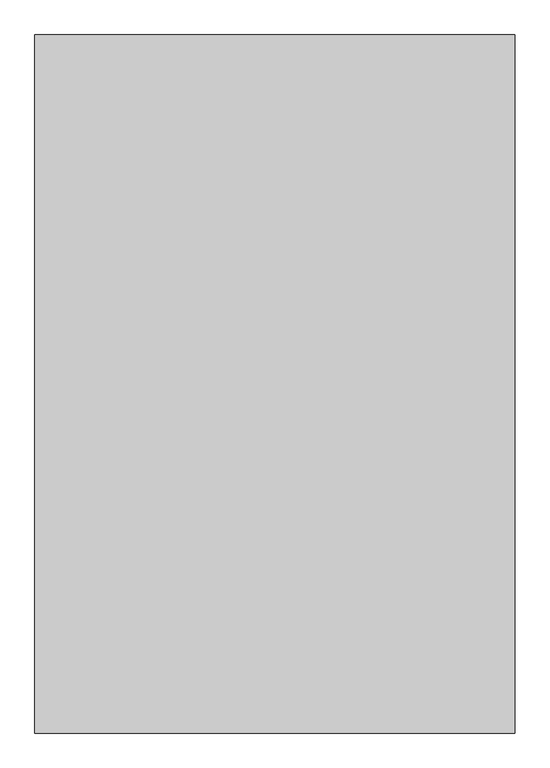
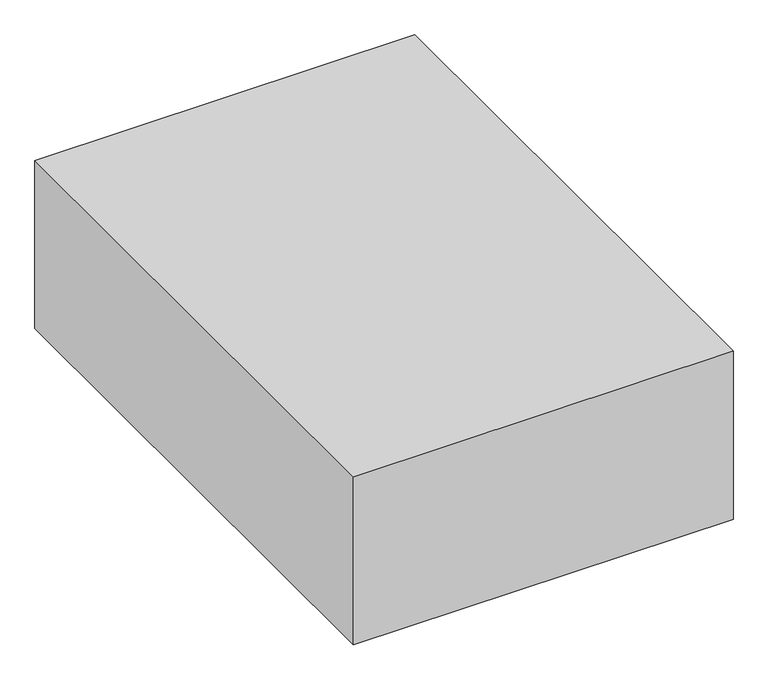
"""IFC4 building model written with IfcOpenShell, lengths in millimetres: proxy geometry, Space Planning Box_hec : Space Planning Box_hec."""

from ifc_helpers import new_model, si_unit, origin, origin_with_axes, place, context, project, spatial, polyline, outline, extrude, source, transform, mapped, element, save


def generic_models_21711933(model_context):
    return source(origin(), model_context, "Body", "SweptSolid", [
        extrude(outline(polyline([(6400.0, 9300.0), (6400.0, -9300.0), (-6400.0, -9300.0), (-6400.0, 9300.0), (6400.0, 9300.0)])), origin_with_axes(), (0.0, 0.0, 1.0), 6000.0),
    ])


if __name__ == "__main__":
    model = new_model("IFC4")
    model_context = context("Model", 3, world=origin())
    ifc_project = project(units=[si_unit("LENGTHUNIT", "METRE", prefix="MILLI")], contexts=[model_context])
    site = spatial("IfcSite", under=ifc_project)
    building = spatial("IfcBuilding", under=site)
    placement = place(None, origin())
    generic_models_shape = generic_models_21711933(model_context)
    element("IfcBuildingElementProxy", 1, Name="Space Planning Box_hec : Space Planning Box_hec", ObjectType="Space Planning Box_hec : Space Planning Box_hec", at=placement, inside=building, context=model_context, shape_type="MappedRepresentation", body=[
        mapped(generic_models_shape, transform((0.0, 0.0, 0.0), x_axis=(1.0, 0.0, 0.0), y_axis=(0.0, 1.0, 0.0), z_axis=(0.0, 0.0, 1.0))),
    ])
    save(model, "model.ifc")

# Revit data of these elements
# Type "Space Planning Box_hec : Space Planning Box_hec"
#   Type Comments = "..."
#   Room Name [instance default] = "?"
#   Interior Finish [instance default] = ""
#   Exterior Finish [instance default] = ""
#   Department [instance default] = ""
#   Assembly Code = "..."
#   Width [instance default] = 1524 mm
#   Program Area [instance default] = 0 m²
#   Length [instance default] = 1524 mm
#   Height [instance default] = 1524 mm
#   Area [instance default] = 2.32258 m²
#   Fill Color [instance default] = Cyan
#   Default Elevation = 0
# Element 1 (IfcBuildingElementProxy, "Space Planning Box_hec : Space Planning Box_hec")
#   Room Name = "Electrical Room"
#   Interior Finish = "IF1"
#   Exterior Finish = "EF1"
#   Department = "EL"
#   Width = 12800 mm
#   Program Area = 238.08 m²
#   Length = 18600 mm
#   Height = 6000 mm
#   Area = 238.08 m²
#   Fill Color = Blue
#   Materials on its faces: "Blue"
# Materials
#   "Cyan": class "Generic", colour RGB 0 255 255, transparency 0.2, Cost = 0
#   "Blue": class "Generic", colour RGB 0 0 255, transparency 0.2, Cost = 0
